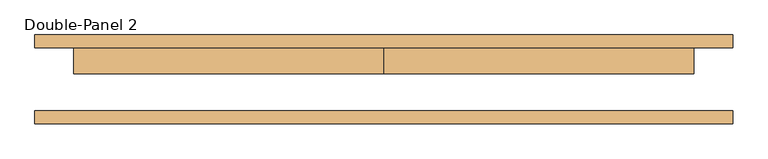
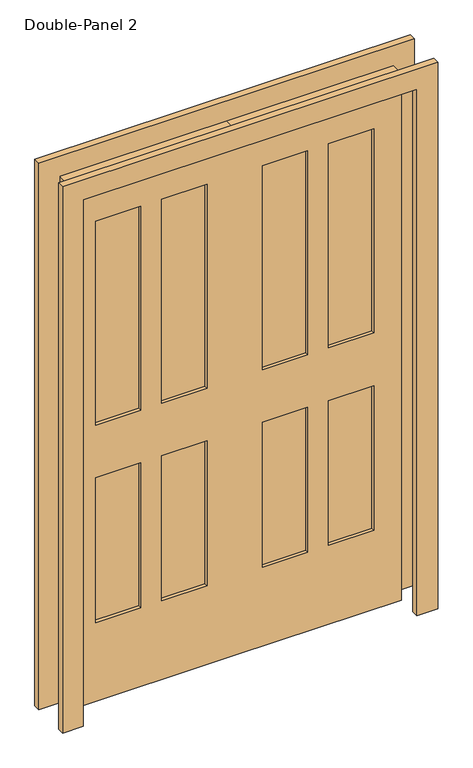
"""IFC4 building model written with IfcOpenShell, lengths in millimetres: door geometry, Double-Panel 2."""

from ifc_helpers import new_model, si_unit, frame, origin, place, context, project, spatial, polyline, outline, extrude, source, transform, mapped, element, save


def double_panel_2_ff92538c(model_context):
    return source(origin(), model_context, "Body", "SweptSolid", [
        extrude(outline(polyline([(2108.2, -685.8), (0.0, -685.8), (0.0, -609.6), (2032.0, -609.6), (2032.0, 609.6), (0.0, 609.6), (0.0, 685.8), (2108.2, 685.8), (2108.2, -685.8)])), frame((0.0, 61.9125, 0.0), z_axis=(0.0, 1.0, 0.0), x_axis=(0.0, 0.0, 1.0)), (0.0, 0.0, 1.0), 25.4),
        extrude(outline(polyline([(342.9, 49.2125), (508.0, 49.2125), (508.0, 23.8125), (342.9, 23.8125), (342.9, 49.2125)])), frame((0.0, 0.0, 1066.8), z_axis=(0.0, 0.0, 1.0), x_axis=(1.0, 0.0, 0.0)), (0.0, 0.0, 1.0), 787.4),
        extrude(outline(polyline([(101.6, 49.2125), (266.7, 49.2125), (266.7, 23.8125), (101.6, 23.8125), (101.6, 49.2125)])), frame((0.0, 0.0, 1066.8), z_axis=(0.0, 0.0, 1.0), x_axis=(1.0, 0.0, 0.0)), (0.0, 0.0, 1.0), 787.4),
        extrude(outline(polyline([(342.9, 49.2125), (508.0, 49.2125), (508.0, 23.8125), (342.9, 23.8125), (342.9, 49.2125)])), frame((0.0, 0.0, 304.8), z_axis=(0.0, 0.0, 1.0), x_axis=(1.0, 0.0, 0.0)), (0.0, 0.0, 1.0), 558.8),
        extrude(outline(polyline([(101.6, 49.2125), (266.7, 49.2125), (266.7, 23.8125), (101.6, 23.8125), (101.6, 49.2125)])), frame((0.0, 0.0, 304.8), z_axis=(0.0, 0.0, 1.0), x_axis=(1.0, 0.0, 0.0)), (0.0, 0.0, 1.0), 558.8),
        extrude(outline(polyline([(-266.7, 49.2125), (-101.6, 49.2125), (-101.6, 23.8125), (-266.7, 23.8125), (-266.7, 49.2125)])), frame((0.0, 0.0, 1066.8), z_axis=(0.0, 0.0, 1.0), x_axis=(1.0, 0.0, 0.0)), (0.0, 0.0, 1.0), 787.4),
        extrude(outline(polyline([(-508.0, 49.2125), (-342.9, 49.2125), (-342.9, 23.8125), (-508.0, 23.8125), (-508.0, 49.2125)])), frame((0.0, 0.0, 1066.8), z_axis=(0.0, 0.0, 1.0), x_axis=(1.0, 0.0, 0.0)), (0.0, 0.0, 1.0), 787.4),
        extrude(outline(polyline([(-266.7, 49.2125), (-101.6, 49.2125), (-101.6, 23.8125), (-266.7, 23.8125), (-266.7, 49.2125)])), frame((0.0, 0.0, 304.8), z_axis=(0.0, 0.0, 1.0), x_axis=(1.0, 0.0, 0.0)), (0.0, 0.0, 1.0), 558.8),
        extrude(outline(polyline([(-508.0, 49.2125), (-342.9, 49.2125), (-342.9, 23.8125), (-508.0, 23.8125), (-508.0, 49.2125)])), frame((0.0, 0.0, 304.8), z_axis=(0.0, 0.0, 1.0), x_axis=(1.0, 0.0, 0.0)), (0.0, 0.0, 1.0), 558.8),
        extrude(outline(polyline([(2032.0, 0.0), (2032.0, -609.6), (0.0, -609.6), (0.0, 0.0), (0.0, 609.6), (2032.0, 609.6), (2032.0, 0.0)]), holes=[polyline([(1854.2, 342.9), (1854.2, 508.0), (1066.8, 508.0), (1066.8, 342.9), (1854.2, 342.9)]), polyline([(1854.2, 101.6), (1854.2, 266.7), (1066.8, 266.7), (1066.8, 101.6), (1854.2, 101.6)]), polyline([(863.6, 342.9), (863.6, 508.0), (304.8, 508.0), (304.8, 342.9), (863.6, 342.9)]), polyline([(863.6, 101.6), (863.6, 266.7), (304.8, 266.7), (304.8, 101.6), (863.6, 101.6)]), polyline([(1066.8, -266.7), (1854.2, -266.7), (1854.2, -101.6), (1066.8, -101.6), (1066.8, -266.7)]), polyline([(1854.2, -508.0), (1854.2, -342.9), (1066.8, -342.9), (1066.8, -508.0), (1854.2, -508.0)]), polyline([(863.6, -266.7), (863.6, -101.6), (304.8, -101.6), (304.8, -266.7), (863.6, -266.7)]), polyline([(863.6, -508.0), (863.6, -342.9), (304.8, -342.9), (304.8, -508.0), (863.6, -508.0)])]), frame((0.0, 11.1125, 0.0), z_axis=(0.0, 1.0, 0.0), x_axis=(0.0, 0.0, 1.0)), (0.0, 0.0, 1.0), 50.8),
        extrude(outline(polyline([(2032.0, -609.6), (2032.0, 609.6), (0.0, 609.6), (0.0, 685.8), (2108.2, 685.8), (2108.2, -685.8), (0.0, -685.8), (0.0, -609.6), (2032.0, -609.6)])), frame((0.0, -87.3125, 0.0), z_axis=(0.0, 1.0, 0.0), x_axis=(0.0, 0.0, 1.0)), (0.0, 0.0, 1.0), 25.4),
    ])


if __name__ == "__main__":
    model = new_model("IFC4")
    model_context = context("Model", 3, world=origin())
    ifc_project = project(units=[si_unit("LENGTHUNIT", "METRE", prefix="MILLI")], contexts=[model_context])
    site = spatial("IfcSite", under=ifc_project)
    building = spatial("IfcBuilding", under=site)
    placement = place(None, origin())
    double_panel_2_shape = double_panel_2_ff92538c(model_context)
    element("IfcDoor", 1, ObjectType="Double-Panel 2 : 48\" x 80\"  White", at=placement, inside=building, context=model_context, shape_type="MappedRepresentation", body=[
        mapped(double_panel_2_shape, transform((0.0, 0.0, 0.0), x_axis=(1.0, 0.0, 0.0), y_axis=(0.0, 1.0, 0.0), z_axis=(0.0, 0.0, 1.0))),
    ])
    save(model, "model.ifc")

# Revit data of these elements
# Type "Double-Panel 2 : 48\" x 80\"  White"
#   Type Mark = "84"
#   COBie.Type.CreatedBy = "doug.wood@us.ibm.com"
#   COBie.Type.CreatedOn = "2016-04-14T02:07:24"
#   COBie.Type.Name = "Doors_Double-Panel 2_48\" x 80\"  White_84"
#   COBie.Type.Category = "23-30 10 00 : Doors"
#   COBie.Type.Description = "Double-Panel 2_48\" x 80\"  White"
#   COBie.Type.Manufacturer = ""
#   COBie.Type.ModelNumber = ""
#   Construction Type Id = "MDOOR"
#   Assembly Code = "C1020"
#   Analytic Construction = "Metal"
#   COBie.Type.ReplacementCost = 0
#   Thickness = 0' - 2"
#   Heat Transfer Coefficient (U) = 3.7021 W/(m²·K)
#   Height = 6' - 8"
#   Trim Projection Ext = 0' - 1"
#   Trim Projection Int = 0' - 1"
#   Trim Width = 0' - 3"
#   Width = 4' - 0"
#   COBie.Type = no
#   Door Material = Door - Panel - White
#   Frame Material = Door - Frame - White
#   Visual Light Transmittance = 0
#   Solar Heat Gain Coefficient = 0
#   Function = (empty or 0)
#   Wall Closure = (empty or 0)
# Element 1 (IfcDoor, "Double-Panel 2 : 48\" x 80\"  White")
#   Materials on its faces: "Door - Panel - White", "Door - Frame - White"
# Materials
#   "Door - Panel - White": class "Wood", colour RGB 255 255 255, transparency 0, Cost = 0
#   "Door - Frame - White": class "Miscellaneous", colour RGB 255 255 255, transparency 0, Cost = 0
